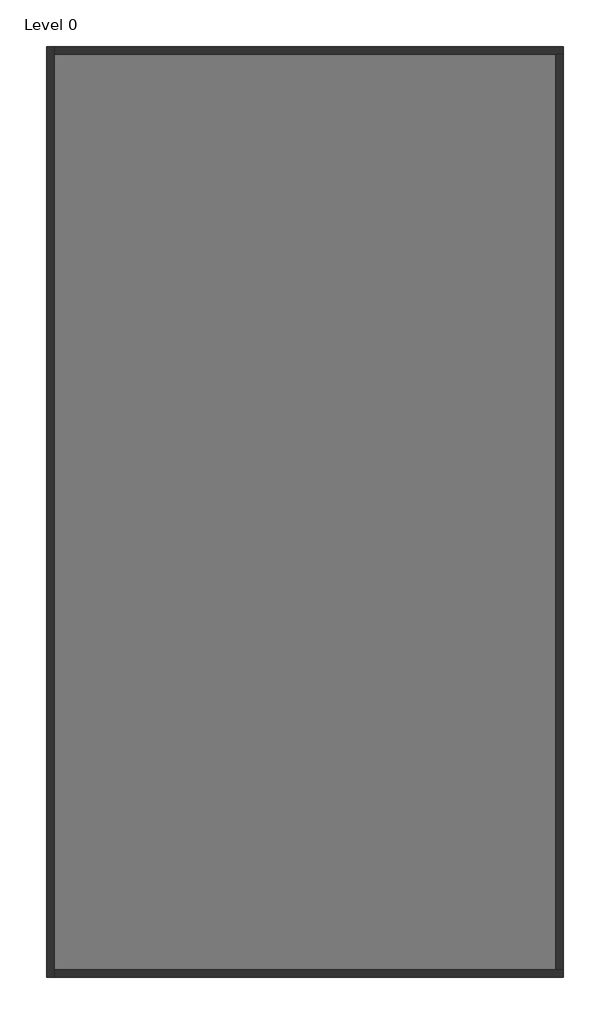
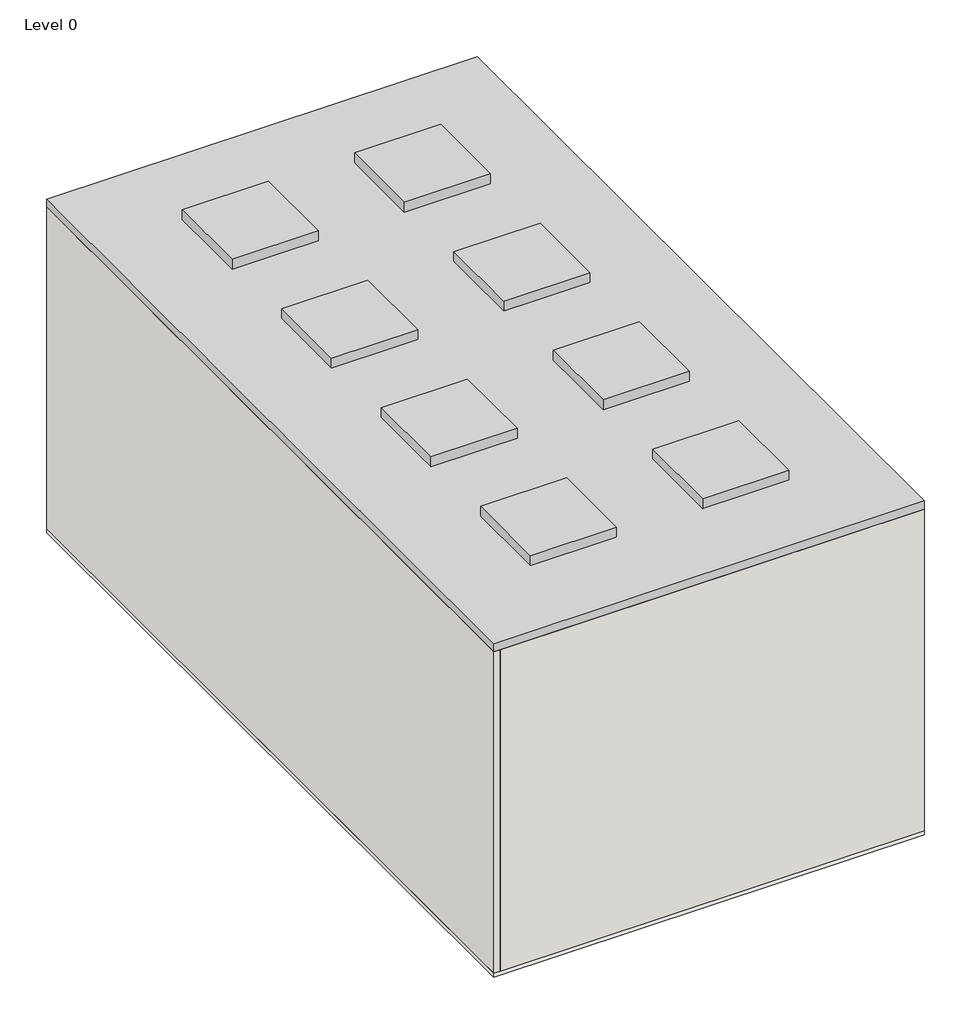
# One storey: 4 walls, 1 proxy, 1 slab.
"""IFC4 building model written with IfcOpenShell, lengths in millimetres."""

from ifc_helpers import new_model, si_unit, frame, origin, origin_with_axes, place, context, project, spatial, polyline, outline, extrude, faceted_brep, element, save

model = new_model("IFC4")

# Units and contexts
model_context = context("Model", 3, world=origin())
ifc_project = project(units=[si_unit("LENGTHUNIT", "METRE", prefix="MILLI")], contexts=[model_context])

# Site, building, storey
site = spatial("IfcSite", under=ifc_project)
building = spatial("IfcBuilding", under=site)
storey = spatial("IfcBuildingStorey", under=building, Name="Level 0", Elevation=100.0)

# Proxy
placement = place(None, origin())
element("IfcBuildingElementProxy", 1, Name="LowUrbanDensityBuilding : LowUrbanDensityBuilding", ObjectType="LowUrbanDensityBuilding : LowUrbanDensityBuilding", at=placement, inside=storey, context=model_context, shape_type="SweptSolid", body=[
    extrude(outline(polyline([(7325.2659446, 3676.2074539), (7325.2659446, -14323.7925461), (-2674.7340554, -14323.7925461), (-2674.7340554, 3676.2074539), (7325.2659446, 3676.2074539)])), origin_with_axes(), (0.0, 0.0, 1.0), 8200.0),
    extrude(outline(polyline([(1325.2659446, 1676.2074539), (1325.2659446, -323.7925461), (-674.7340554, -323.7925461), (-674.7340554, 1676.2074539), (1325.2659446, 1676.2074539)])), frame((0.0, 0.0, 8200.0), z_axis=(0.0, 0.0, 1.0), x_axis=(1.0, 0.0, 0.0)), (0.0, 0.0, 1.0), 245.0),
    extrude(outline(polyline([(5325.2659446, 1676.2074539), (5325.2659446, -323.7925461), (3325.2659446, -323.7925461), (3325.2659446, 1676.2074539), (5325.2659446, 1676.2074539)])), frame((0.0, 0.0, 8200.0), z_axis=(0.0, 0.0, 1.0), x_axis=(1.0, 0.0, 0.0)), (0.0, 0.0, 1.0), 245.0),
    extrude(outline(polyline([(1325.2659446, -2323.7925461), (1325.2659446, -4323.7925461), (-674.7340554, -4323.7925461), (-674.7340554, -2323.7925461), (1325.2659446, -2323.7925461)])), frame((0.0, 0.0, 8200.0), z_axis=(0.0, 0.0, 1.0), x_axis=(1.0, 0.0, 0.0)), (0.0, 0.0, 1.0), 245.0),
    extrude(outline(polyline([(5325.2659446, -2323.7925461), (5325.2659446, -4323.7925461), (3325.2659446, -4323.7925461), (3325.2659446, -2323.7925461), (5325.2659446, -2323.7925461)])), frame((0.0, 0.0, 8200.0), z_axis=(0.0, 0.0, 1.0), x_axis=(1.0, 0.0, 0.0)), (0.0, 0.0, 1.0), 245.0),
    extrude(outline(polyline([(1325.2659446, -6323.7925461), (1325.2659446, -8323.7925461), (-674.7340554, -8323.7925461), (-674.7340554, -6323.7925461), (1325.2659446, -6323.7925461)])), frame((0.0, 0.0, 8200.0), z_axis=(0.0, 0.0, 1.0), x_axis=(1.0, 0.0, 0.0)), (0.0, 0.0, 1.0), 245.0),
    extrude(outline(polyline([(5325.2659446, -6323.7925461), (5325.2659446, -8323.7925461), (3325.2659446, -8323.7925461), (3325.2659446, -6323.7925461), (5325.2659446, -6323.7925461)])), frame((0.0, 0.0, 8200.0), z_axis=(0.0, 0.0, 1.0), x_axis=(1.0, 0.0, 0.0)), (0.0, 0.0, 1.0), 245.0),
    extrude(outline(polyline([(1325.2659446, -10323.7925461), (1325.2659446, -12323.7925461), (-674.7340554, -12323.7925461), (-674.7340554, -10323.7925461), (1325.2659446, -10323.7925461)])), frame((0.0, 0.0, 8200.0), z_axis=(0.0, 0.0, 1.0), x_axis=(1.0, 0.0, 0.0)), (0.0, 0.0, 1.0), 245.0),
    extrude(outline(polyline([(5325.2659446, -10323.7925461), (5325.2659446, -12323.7925461), (3325.2659446, -12323.7925461), (3325.2659446, -10323.7925461), (5325.2659446, -10323.7925461)])), frame((0.0, 0.0, 8200.0), z_axis=(0.0, 0.0, 1.0), x_axis=(1.0, 0.0, 0.0)), (0.0, 0.0, 1.0), 245.0),
])

# Slab
element("IfcSlab", 2, ObjectType="Floor-Concrete_100Con", at=placement, inside=storey, context=model_context, shape_type="SweptSolid", body=[
    extrude(outline(polyline([(7325.2659446, 3676.2074539), (7325.2659446, -14323.7925461), (-2674.7340554, -14323.7925461), (-2674.7340554, 3676.2074539), (7325.2659446, 3676.2074539)])), origin_with_axes(), (0.0, 0.0, 1.0), 100.0),
])

# Walls
element("IfcWall", 3, ObjectType="Wall-Ext_25Rdr-100Blk-19P", at=placement, inside=storey, context=model_context, shape_type="Brep", body=[
    faceted_brep([(-2674.7340554, 3676.2074539, 100.0), (-2674.7340554, -14323.7925461, 100.0), (-2674.7340554, -14323.7925461, 8000.0), (-2674.7340554, 3676.2074539, 8000.0), (-2530.4340554, 3676.2074539, 100.0), (-2530.4340554, 3676.2074539, 8000.0), (-2530.4340554, 3531.9074539, 8000.0), (-2530.4340554, -14179.4925461, 8000.0), (-2530.4340554, -14323.7925461, 8000.0), (-2530.4340554, -14323.7925461, 100.0), (-2530.4340554, -14179.4925461, 100.0), (-2530.4340554, 3531.9074539, 100.0)], [[[0, 1, 2, 3]], [[4, 5, 6, 7, 8, 9, 10, 11]], [[1, 0, 4, 11, 10, 9]], [[3, 2, 8, 7, 6, 5]], [[2, 1, 9, 8]], [[0, 3, 5, 4]]]),
])
element("IfcWall", 4, ObjectType="Wall-Ext_25Rdr-100Blk-19P", at=placement, inside=storey, context=model_context, shape_type="Brep", body=[
    faceted_brep([(-2530.4340554, -14323.7925461, 100.0), (7325.2659446, -14323.7925461, 100.0), (7325.2659446, -14323.7925461, 8000.0), (-2530.4340554, -14323.7925461, 8000.0), (-2530.4340554, -14179.4925461, 100.0), (-2530.4340554, -14179.4925461, 8000.0), (7180.9659446, -14179.4925461, 8000.0), (7325.2659446, -14179.4925461, 8000.0), (7325.2659446, -14179.4925461, 100.0), (7180.9659446, -14179.4925461, 100.0)], [[[0, 1, 2, 3]], [[4, 5, 6, 7, 8, 9]], [[1, 0, 4, 9, 8]], [[3, 2, 7, 6, 5]], [[0, 3, 5, 4]], [[2, 1, 8, 7]]]),
])
element("IfcWall", 5, ObjectType="Wall-Ext_25Rdr-100Blk-19P", at=placement, inside=storey, context=model_context, shape_type="Brep", body=[
    faceted_brep([(7325.2659446, 3676.2074539, 100.0), (-2530.4340554, 3676.2074539, 100.0), (-2530.4340554, 3676.2074539, 8000.0), (7325.2659446, 3676.2074539, 8000.0), (7325.2659446, 3531.9074539, 100.0), (7325.2659446, 3531.9074539, 8000.0), (7180.9659446, 3531.9074539, 8000.0), (-2530.4340554, 3531.9074539, 8000.0), (-2530.4340554, 3531.9074539, 100.0), (7180.9659446, 3531.9074539, 100.0)], [[[0, 1, 2, 3]], [[4, 5, 6, 7, 8, 9]], [[1, 0, 4, 9, 8]], [[3, 2, 7, 6, 5]], [[2, 1, 8, 7]], [[0, 3, 5, 4]]]),
])
element("IfcWall", 6, ObjectType="Wall-Ext_25Rdr-100Blk-19P", at=placement, inside=storey, context=model_context, shape_type="SweptSolid", body=[
    extrude(outline(polyline([(7325.2659446, 3531.9074539), (7325.2659446, -14179.4925461), (7180.9659446, -14179.4925461), (7180.9659446, 3531.9074539), (7325.2659446, 3531.9074539)])), frame((0.0, 0.0, 100.0), z_axis=(0.0, 0.0, 1.0), x_axis=(1.0, 0.0, 0.0)), (0.0, 0.0, 1.0), 7900.0),
])

save(model, "model.ifc")

# Revit data of these elements
# Project information
#   Project Issue Date = "Issue Date"
#   Project Status = "Project Status"
#   Client Name = "Owner"
#   Project Address = "Enter address here"
#   Project Name = "Project Name"
#   Project Number = "Project Number"
# Type "Floor-Concrete_100Con"
#   Keynote = "E60/130"
#   Function = 0
#   Layers, outside or top first: 100 mm "Concrete" (function 1)
# Type "Wall-Ext_25Rdr-100Blk-19P"
#   Keynote = "F10"
#   Layers, outside or top first: 25.3 mm "Render, Beige, Smooth" (function 5); 100 mm "Concrete Masonry Units _Low Density" (function 1); 19 mm "Plaster" (function 5)
# Element 1 (IfcBuildingElementProxy, "LowUrbanDensityBuilding : LowUrbanDensityBuilding")
#   Phase Created = New Construction
#   Materials on its faces: "Default Form"
# Element 2 (IfcSlab, "Floor-Concrete_100Con")
#   Height Offset From Level = 0 mm
#   Phase Created = New Construction
#   Materials on its faces: "Concrete"
# Element 3 (IfcWall, "Wall-Ext_25Rdr-100Blk-19P")
#   Top Offset = 0 mm
#   Base Offset = 0 mm
#   wall height = 7900 mm
#   Phase Created = New Construction
#   Base Constraint = Level 0
#   Top Constraint = Level 2
#   Materials on its faces: "Render, Beige, Smooth", "Default Wall", "Plaster"
# Elements 4, 5, 6 (IfcWall, "Wall-Ext_25Rdr-100Blk-19P")
#   Top Offset = 0 mm
#   Base Offset = 0 mm
#   wall height = 7900 mm
#   Phase Created = New Construction
#   Base Constraint = Level 0
#   Top Constraint = Level 2
#   Materials on its faces: "Default Wall", "Render, Beige, Smooth", "Plaster"
# Materials
#   "Concrete": class "Concrete", colour RGB 120 120 120, transparency 0, Description = "Portland Cement Concrete", Cost = 0
#   "Render, Beige, Smooth": class "Generic", colour RGB 213 198 180, transparency 0, Description = "physical material", Cost = 0
#   "Concrete Masonry Units _Low Density": class "Masonry", colour RGB 181 181 181, transparency 0, Description = "Concrete masonry units", Cost = 0
#   "Plaster": class "Generic", colour RGB 249 249 249, transparency 0, Description = "Plaster", Cost = 0
#   "Default Form": class "Generic", colour RGB 185 189 196, transparency 0.5, Cost = 0
#   "Default Wall": class "Miscellaneous", colour RGB 128 128 128, transparency 0, Comments = "Rendering appearance not upgraded Rendering appearance not upgraded ", Cost = 0
